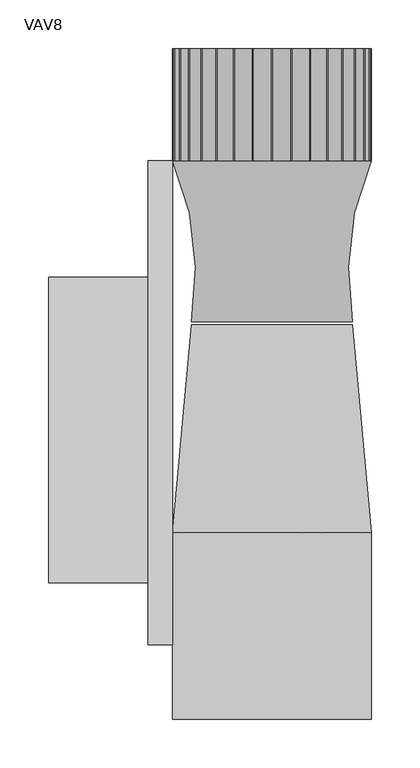
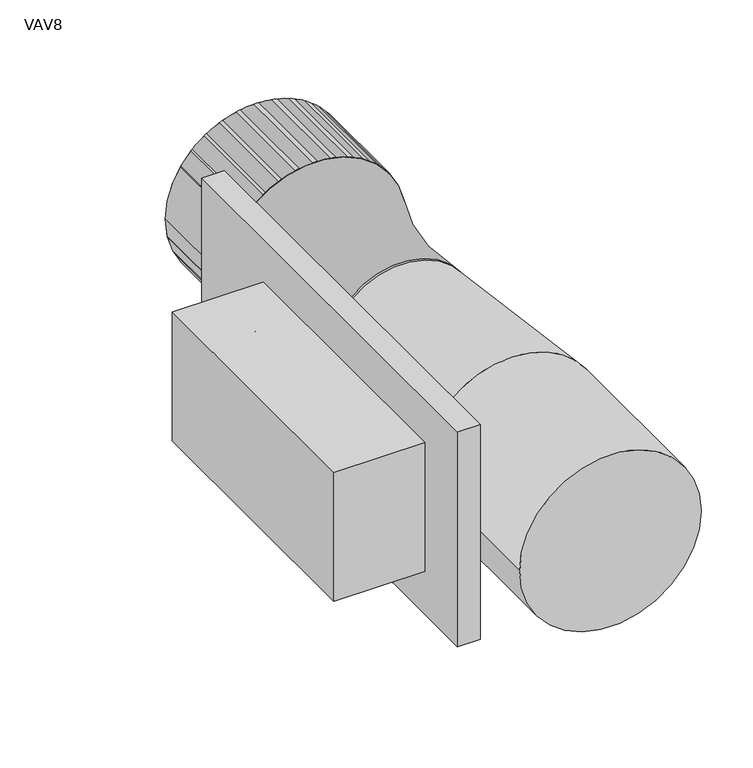
"""IFC4 building model written with IfcOpenShell, lengths in millimetres: proxy geometry, VAV8 : PValve200."""

import ifcopenshell
import ifcopenshell.guid

model = None  # the IFC model being written
_history = None  # IfcOwnerHistory: only IFC2X3 demands one
_inside = {}  # id of a spatial element -> (the spatial element, [elements in it])
_under = {}  # id of a project, library or spatial element -> (it, [spatial elements below it])
_declared = {}  # id of a project -> (the project, [libraries it declares])
_typed = {}  # id of a type object -> (the type object, [elements of that type])
_made_of = {}  # id of a material, layer set ... -> (it, [elements and type objects made of it])


def new_model(schema):
    """Start an empty IFC model of exactly this schema.

    Asked for "IFC4X3", IfcOpenShell would pick the latest addendum, in which some entities
    have other attributes; the version numbers below select the first issue.
    IFC2X3 requires an IfcOwnerHistory on every rooted entity: one is made here for all.
    """
    global model, _history
    if schema == "IFC4X3":
        model = ifcopenshell.file(schema_version=(4, 3, 0, 0))
    else:
        model = ifcopenshell.file(schema=schema)
    _inside.clear()
    _under.clear()
    _declared.clear()
    _typed.clear()
    _made_of.clear()
    _history = None
    if model.schema == "IFC2X3":
        org = make("IfcOrganization", Name="unknown")
        user = make(
            "IfcPersonAndOrganization",
            ThePerson=make("IfcPerson", FamilyName="unknown"),
            TheOrganization=org,
        )
        app = make(
            "IfcApplication",
            ApplicationDeveloper=org,
            Version="unknown",
            ApplicationFullName="unknown",
            ApplicationIdentifier="unknown",
        )
        _history = make(
            "IfcOwnerHistory",
            OwningUser=user,
            OwningApplication=app,
            ChangeAction="ADDED",
            CreationDate=0,
        )
    return model


def make(cls, **values):
    """One entity of the class cls with the attributes given. An attribute that is None is left unset."""
    return model.create_entity(
        cls, **{name: value for name, value in values.items() if value is not None}
    )


def rooted(cls, **values):
    """An entity with a GlobalId (a new one), such as an element, a storey or a relation."""
    return make(cls, GlobalId=ifcopenshell.guid.new(), OwnerHistory=_history, **values)


def si_unit(unit_type, name, prefix=None):
    """IfcSIUnit, for example si_unit("LENGTHUNIT", "METRE", prefix="MILLI")."""
    return make("IfcSIUnit", UnitType=unit_type, Prefix=prefix, Name=name)


def assignment(units):
    """IfcUnitAssignment: the units of a project."""
    return None if units is None else make("IfcUnitAssignment", Units=units)


def point(xyz):
    """IfcCartesianPoint."""
    return None if xyz is None else make("IfcCartesianPoint", Coordinates=xyz)


def direction(xyz):
    """IfcDirection."""
    return None if xyz is None else make("IfcDirection", DirectionRatios=xyz)


def frame(location, z_axis=None, x_axis=None):
    """IfcAxis2Placement3D, a coordinate frame: its origin and axes. An axis left out is left unset."""
    return make(
        "IfcAxis2Placement3D",
        Location=point(location),
        Axis=direction(z_axis),
        RefDirection=direction(x_axis),
    )


def frame_2d(location, x_axis=None):
    """IfcAxis2Placement2D, a coordinate frame in the plane: its origin and x axis."""
    return make(
        "IfcAxis2Placement2D", Location=point(location), RefDirection=direction(x_axis)
    )


def origin():
    """The frame at (0, 0, 0) with its axes left unset."""
    return frame((0.0, 0.0, 0.0))


def origin_2d():
    """The frame at (0, 0) in the plane with its x axis left unset."""
    return frame_2d((0.0, 0.0))


def place(relative_to, where):
    """IfcLocalPlacement: puts the frame where relative to a parent placement (None: the world)."""
    return make(
        "IfcLocalPlacement", PlacementRelTo=relative_to, RelativePlacement=where
    )


def context(
    kind, dimensions, precision=None, world=None, true_north=None, identifier=None
):
    """IfcGeometricRepresentationContext, for example the 3D "Model" context."""
    return make(
        "IfcGeometricRepresentationContext",
        ContextIdentifier=identifier,
        ContextType=kind,
        CoordinateSpaceDimension=dimensions,
        Precision=precision,
        WorldCoordinateSystem=world,
        TrueNorth=true_north,
    )


def project(units=None, contexts=None):
    """IfcProject with its units and contexts."""
    return rooted(
        "IfcProject",
        Name="project",
        RepresentationContexts=contexts,
        UnitsInContext=assignment(units),
    )


def spatial(cls, under=None, at=None, **own):
    """A site, building, storey or space (cls), placed at a placement, below another one or the project."""
    s = rooted(cls, ObjectPlacement=at, **own)
    if under is not None:
        _under.setdefault(under.id(), (under, []))[1].append(s)
    return s


def polyline(points):
    """IfcPolyline through the points."""
    return make("IfcPolyline", Points=[point(p) for p in points])


def circle_curve(where, radius):
    """IfcCircle in the frame where."""
    return make("IfcCircle", Position=where, Radius=radius)


def ellipse_curve(where, semi_axis1, semi_axis2):
    """IfcEllipse in the frame where."""
    return make(
        "IfcEllipse", Position=where, SemiAxis1=semi_axis1, SemiAxis2=semi_axis2
    )


def trimmed(basis, trim1, trim2, sense, master):
    """IfcTrimmedCurve: the piece of a basis curve between two trims."""
    return make(
        "IfcTrimmedCurve",
        BasisCurve=basis,
        Trim1=trim1,
        Trim2=trim2,
        SenseAgreement=sense,
        MasterRepresentation=master,
    )


def segment(curve, same_sense, transition):
    """IfcCompositeCurveSegment."""
    return make(
        "IfcCompositeCurveSegment",
        Transition=transition,
        SameSense=same_sense,
        ParentCurve=curve,
    )


def composite_curve(segments, self_intersect=None):
    """IfcCompositeCurve: segments joined end to end."""
    return make("IfcCompositeCurve", Segments=segments, SelfIntersect=self_intersect)


def outline(outer, holes=None, kind="AREA"):
    """IfcArbitraryClosedProfileDef: a profile drawn as a closed curve; with holes, ...WithVoids."""
    if holes is None:
        return make("IfcArbitraryClosedProfileDef", ProfileType=kind, OuterCurve=outer)
    return make(
        "IfcArbitraryProfileDefWithVoids",
        ProfileType=kind,
        OuterCurve=outer,
        InnerCurves=holes,
    )


def extrude(swept, where, along, depth):
    """IfcExtrudedAreaSolid: the profile swept, set in the frame where, extruded along a direction by depth."""
    return make(
        "IfcExtrudedAreaSolid",
        SweptArea=swept,
        Position=where,
        ExtrudedDirection=direction(along),
        Depth=depth,
    )


def shape(context_of_items, identifier, shape_type, items):
    """IfcShapeRepresentation: the items that make up one representation, for example the "Body"."""
    return make(
        "IfcShapeRepresentation",
        ContextOfItems=context_of_items,
        RepresentationIdentifier=identifier,
        RepresentationType=shape_type,
        Items=items,
    )


def source(mapping_origin, context_of_items, identifier, shape_type, items):
    """IfcRepresentationMap: a shape defined once, which mapped items show again and again."""
    return make(
        "IfcRepresentationMap",
        MappingOrigin=mapping_origin,
        MappedRepresentation=shape(context_of_items, identifier, shape_type, items),
    )


def transform(
    local_origin,
    x_axis=None,
    y_axis=None,
    z_axis=None,
    scale=None,
    scale2=None,
    scale3=None,
    uniform=True,
):
    """IfcCartesianTransformationOperator3D, or its non-uniform kind. x_axis, y_axis, z_axis: its Axis1, 2, 3."""
    if uniform:
        return make(
            "IfcCartesianTransformationOperator3D",
            Axis1=direction(x_axis),
            Axis2=direction(y_axis),
            LocalOrigin=point(local_origin),
            Scale=scale,
            Axis3=direction(z_axis),
        )
    return make(
        "IfcCartesianTransformationOperator3DnonUniform",
        Axis1=direction(x_axis),
        Axis2=direction(y_axis),
        LocalOrigin=point(local_origin),
        Scale=scale,
        Axis3=direction(z_axis),
        Scale2=scale2,
        Scale3=scale3,
    )


def mapped(mapping_source, mapping_target):
    """IfcMappedItem: shows the shape of a source again, moved by a transform."""
    return make(
        "IfcMappedItem", MappingSource=mapping_source, MappingTarget=mapping_target
    )


def made_of(thing, what):
    """Note that an element or type object is made of a material, layer set ...; save() writes the relation."""
    if what is not None:
        _made_of.setdefault(what.id(), (what, []))[1].append(thing)
    return thing


def element(
    cls,
    number,
    at=None,
    inside=None,
    cuts=None,
    type_object=None,
    material=None,
    context=None,
    identifier="Body",
    shape_type=None,
    held_by="IfcProductDefinitionShape",
    body=None,
    shapes=None,
    **own,
):
    """One element of the class cls, such as IfcWall. Its Tag is "e" and its number.

    at: its placement. inside: the storey or other place that contains it. cuts: it is an
    opening in that element (IfcRelVoidsElement). A single representation is given by context,
    identifier, shape_type and body (its items); several are given by shapes. held_by: the class
    of the entity that holds the representations. save() writes the other relations.
    """
    e = rooted(cls, Tag="e%d" % number, ObjectPlacement=at, **own)
    if body is not None:
        shapes = [shape(context, identifier, shape_type, body)]
    if shapes is not None:
        e.Representation = make(held_by, Representations=shapes)
    if inside is not None:
        _inside.setdefault(inside.id(), (inside, []))[1].append(e)
    if cuts is not None:
        rooted(
            "IfcRelVoidsElement", RelatingBuildingElement=cuts, RelatedOpeningElement=e
        )
    if type_object is not None:
        _typed.setdefault(type_object.id(), (type_object, []))[1].append(e)
    return made_of(e, material)


def aggregate(whole, parts):
    """IfcRelAggregates: a whole, such as a stair, and the parts it consists of."""
    return rooted("IfcRelAggregates", RelatingObject=whole, RelatedObjects=parts)


def save(model, path):
    """Write the relations noted so far, then the file.

    IfcRelAggregates (storeys below a building ...), IfcRelContainedInSpatialStructure (elements
    in a storey), IfcRelDefinesByType, IfcRelAssociatesMaterial and IfcRelDeclares: one each for
    every whole, place, type object, material and project.
    """
    for whole, parts in _under.values():
        aggregate(whole, parts)
    for where, things in _inside.values():
        rooted(
            "IfcRelContainedInSpatialStructure",
            RelatedElements=things,
            RelatingStructure=where,
        )
    for kind, things in _typed.values():
        rooted("IfcRelDefinesByType", RelatedObjects=things, RelatingType=kind)
    for what, things in _made_of.values():
        rooted("IfcRelAssociatesMaterial", RelatedObjects=things, RelatingMaterial=what)
    for by, libraries in _declared.values():
        rooted("IfcRelDeclares", RelatingContext=by, RelatedDefinitions=libraries)
    model.write(path)


def plane_surface(at):
    """IfcPlane: the flat surface through the origin of the frame at, square to its z axis."""
    return make("IfcPlane", Position=at)


def revolved_surface(curve, axis_point, axis_direction):
    """IfcSurfaceOfRevolution: the curve turned about the line through axis_point along axis_direction."""
    return make(
        "IfcSurfaceOfRevolution",
        SweptCurve=make("IfcArbitraryOpenProfileDef", ProfileType="CURVE", Curve=curve),
        AxisPosition=make("IfcAxis1Placement", Location=point(axis_point), Axis=direction(axis_direction)),
    )


def advanced_brep(points, edges, surfaces, faces):
    """IfcAdvancedBrep: a solid bounded by faces that lie on surfaces and meet in shared edges.

    An edge is (start, end): straight between two places in points (the first is 0);
    or (start, end, curve); or (start, end, curve, False) where it runs against its curve.
    A face is (place in surfaces, loops), or (place, loops, False) where it looks against
    its surface's normal. A loop lists edges by number (the first is 1), with a minus sign
    where the edge is run from its end to its start. The first loop is the outer one.
    """
    corners = [point(p) for p in points]
    vertices = [make("IfcVertexPoint", VertexGeometry=c) for c in corners]
    made = []
    for start, end, *more in edges:
        made.append(
            make(
                "IfcEdgeCurve",
                EdgeStart=vertices[start],
                EdgeEnd=vertices[end],
                EdgeGeometry=more[0] if more else make("IfcPolyline", Points=[corners[start], corners[end]]),
                SameSense=more[1] if len(more) > 1 else True,
            )
        )
    hull = []
    for where, loops, *sense in faces:
        bounds = []
        for j, loop in enumerate(loops):
            ring = [make("IfcOrientedEdge", EdgeElement=made[abs(k) - 1], Orientation=k > 0) for k in loop]
            bounds.append(
                make(
                    "IfcFaceOuterBound" if j == 0 else "IfcFaceBound",
                    Bound=make("IfcEdgeLoop", EdgeList=ring),
                    Orientation=True,
                )
            )
        hull.append(make("IfcAdvancedFace", Bounds=bounds, FaceSurface=surfaces[where], SameSense=sense[0] if sense else True))
    return make("IfcAdvancedBrep", Outer=make("IfcClosedShell", CfsFaces=hull))


def vav8_9bf4b91b(model_context):
    return source(origin(), model_context, "Body", "SolidModel", [
        extrude(outline(composite_curve([segment(trimmed(circle_curve(origin_2d(), 101.6), [point((0.0, 101.6))], [point((0.0, -101.6))], False, "CARTESIAN"), True, "CONTINUOUS"), segment(trimmed(circle_curve(origin_2d(), 101.6), [point((0.0, -101.6))], [point((0.0, 101.6))], False, "CARTESIAN"), True, "CONTINUOUS")], self_intersect=False)), frame((0.0, -114.3, 0.0), z_axis=(0.0, 1.0, 0.0), x_axis=(0.0, 0.0, 1.0)), (0.0, 0.0, 1.0), 114.3),
        advanced_brep(
        [(101.6, -114.3, 0.0), (-101.6, -114.3, 0.0), (-63.5, -114.3, 0.0), (63.5, -114.3, 0.0), (-82.55, -279.4, 0.0), (82.55, -279.4, 0.0), (63.5, -279.4, 0.0), (-63.5, -279.4, 0.0)],
        [
            (0, 1, circle_curve(frame((0.0, -114.3, 0.0), z_axis=(0.0, 1.0, 0.0), x_axis=(1.0, 0.0, 0.0)), 101.6)),
            (1, 2),
            (2, 3, circle_curve(frame((0.0, -114.3, 0.0), z_axis=(0.0, -1.0, 0.0), x_axis=(1.0, 0.0, 0.0)), 63.5)),
            (3, 0),
            (1, 0, circle_curve(frame((0.0, -114.3, 0.0), z_axis=(0.0, 1.0, 0.0), x_axis=(1.0, 0.0, 0.0)), 101.6)),
            (3, 2, circle_curve(frame((0.0, -114.3, 0.0), z_axis=(0.0, -1.0, 0.0), x_axis=(1.0, 0.0, 0.0)), 63.5)),
            (4, 5, circle_curve(frame((0.0, -279.4, 0.0), z_axis=(0.0, -1.0, 0.0), x_axis=(1.0, 0.0, 0.0)), 82.55)),
            (5, 6),
            (6, 7, circle_curve(frame((0.0, -279.4, 0.0), z_axis=(0.0, 1.0, 0.0), x_axis=(1.0, 0.0, 0.0)), 63.5)),
            (7, 4),
            (5, 4, circle_curve(frame((0.0, -279.4, 0.0), z_axis=(0.0, -1.0, 0.0), x_axis=(1.0, 0.0, 0.0)), 82.55)),
            (7, 6, circle_curve(frame((0.0, -279.4, 0.0), z_axis=(0.0, 1.0, 0.0), x_axis=(1.0, 0.0, 0.0)), 63.5)),
            (6, 3),
            (2, 7),
            (0, 5, circle_curve(frame((368.6011377, -228.756862, 0.0), z_axis=(0.0, 0.0, 1.0), x_axis=(1.0, 0.0, 0.0)), 290.4995367)),
            (4, 1, circle_curve(frame((-368.6011377, -228.756862, 0.0), z_axis=(0.0, 0.0, 1.0), x_axis=(-1.0, 0.0, 0.0)), 290.4995367)),
        ],
        [
            plane_surface(frame((0.0, -114.3, 0.0), z_axis=(0.0, 1.0, 0.0), x_axis=(1.0, 0.0, 0.0))),
            plane_surface(frame((0.0, -279.4, 0.0), z_axis=(0.0, -1.0, 0.0), x_axis=(1.0, 0.0, 0.0))),
            revolved_surface(polyline([(63.5, -279.4, 0.0), (63.5, -114.3, 0.0)]), (0.0, 0.0, 0.0), (0.0, -1.0, 0.0)),
            revolved_surface(trimmed(ellipse_curve(frame((368.6011377, -228.756862, 0.0), z_axis=(0.0, 0.0, -1.0), x_axis=(1.0, 0.0, 0.0)), 290.4995367, 290.4995367), [point((82.55, -279.4, 0.0))], [point((101.6, -114.3, 0.0))], True, "CARTESIAN"), (0.0, -114.3, 0.0), (0.0, 1.0, 0.0)),
        ],
        [
            (0, [[1, 2, 3, 4]]),
            (0, [[5, -4, 6, -2]]),
            (1, [[7, 8, 9, 10]]),
            (1, [[11, -10, 12, -8]]),
            (2, [[13, -3, 14, -9]]),
            (2, [[-13, -12, -14, -6]]),
            (3, [[-1, 15, -7, 16]]),
            (3, [[-5, -16, -11, -15]]),
        ],
    ),
        extrude(outline(composite_curve([segment(trimmed(circle_curve(origin_2d(), 101.6), [point((0.0, -101.6))], [point((0.0, 101.6))], False, "CARTESIAN"), True, "CONTINUOUS"), segment(trimmed(circle_curve(origin_2d(), 101.6), [point((0.0, 101.6))], [point((0.0, -101.6))], False, "CARTESIAN"), True, "CONTINUOUS")], self_intersect=False), holes=[composite_curve([segment(trimmed(circle_curve(origin_2d(), 63.5), [point((0.0, 63.5))], [point((0.0, -63.5))], True, "CARTESIAN"), True, "CONTINUOUS"), segment(trimmed(circle_curve(origin_2d(), 63.5), [point((0.0, -63.5))], [point((0.0, 63.5))], True, "CARTESIAN"), True, "CONTINUOUS")], self_intersect=False)]), frame((0.0, -114.3, 0.0), z_axis=(0.0, 1.0, 0.0), x_axis=(0.0, 0.0, 1.0)), (0.0, 0.0, 1.0), 114.3),
        extrude(outline(polyline([(-228.6, -546.1), (-228.6, -233.5601781), (-127.0, -233.5601781), (-127.0, -546.1), (-228.6, -546.1)])), frame((0.0, 0.0, -76.2), z_axis=(0.0, 0.0, 1.0), x_axis=(1.0, 0.0, 0.0)), (0.0, 0.0, 1.0), 152.4),
        extrude(outline(polyline([(-101.6, -609.6), (-127.0, -609.6), (-127.0, -114.3), (-101.6, -114.3), (-101.6, -609.6)])), frame((0.0, 0.0, -127.0), z_axis=(0.0, 0.0, 1.0), x_axis=(1.0, 0.0, 0.0)), (0.0, 0.0, 1.0), 254.0),
        extrude(outline(composite_curve([segment(trimmed(circle_curve(origin_2d(), 101.6), [point((0.0, -101.6))], [point((0.0, 101.6))], False, "CARTESIAN"), True, "CONTINUOUS"), segment(trimmed(circle_curve(origin_2d(), 101.6), [point((0.0, 101.6))], [point((0.0, -101.6))], False, "CARTESIAN"), True, "CONTINUOUS")], self_intersect=False)), frame((0.0, -685.8, 0.0), z_axis=(0.0, 1.0, 0.0), x_axis=(0.0, 0.0, 1.0)), (0.0, 0.0, 1.0), 190.5),
        advanced_brep(
        [(0.0, -495.3, 0.0), (-101.6, -495.3, 0.0), (101.6, -495.3, 0.0), (82.55, -282.3810845, 0.0), (-82.55, -282.3810845, 0.0), (0.0, -282.3810845, 0.0)],
        [
            (0, 1),
            (1, 2, circle_curve(frame((0.0, -495.3, 0.0), z_axis=(0.0, -1.0, 0.0), x_axis=(-1.0, 0.0, 0.0)), 101.6)),
            (2, 0),
            (2, 1, circle_curve(frame((0.0, -495.3, 0.0), z_axis=(0.0, -1.0, 0.0), x_axis=(-1.0, 0.0, 0.0)), 101.6)),
            (3, 4, circle_curve(frame((0.0, -282.3810845, 0.0), z_axis=(0.0, 1.0, 0.0), x_axis=(-1.0, 0.0, 0.0)), 82.55)),
            (4, 5),
            (5, 3),
            (4, 3, circle_curve(frame((0.0, -282.3810845, 0.0), z_axis=(0.0, 1.0, 0.0), x_axis=(-1.0, 0.0, 0.0)), 82.55)),
            (1, 4),
            (3, 2),
        ],
        [
            plane_surface(frame((0.0, -495.3, 0.0), z_axis=(0.0, -1.0, 0.0), x_axis=(-1.0, 0.0, 0.0))),
            plane_surface(frame((0.0, -282.3810845, 0.0), z_axis=(0.0, 1.0, 0.0), x_axis=(-1.0, 0.0, 0.0))),
            revolved_surface(polyline([(-82.55, -282.3810845, 0.0), (-101.6, -495.3, 0.0)]), (0.0, -279.4, 0.0), (0.0, -1.0, 0.0)),
        ],
        [
            (0, [[1, 2, 3]]),
            (0, [[-3, 4, -1]]),
            (1, [[5, 6, 7]]),
            (1, [[8, -7, -6]]),
            (2, [[-2, 9, -5, 10]]),
            (2, [[-4, -10, -8, -9]]),
        ],
    ),
    ])


if __name__ == "__main__":
    model = new_model("IFC4")
    model_context = context("Model", 3, world=origin())
    ifc_project = project(units=[si_unit("LENGTHUNIT", "METRE", prefix="MILLI")], contexts=[model_context])
    site = spatial("IfcSite", under=ifc_project)
    building = spatial("IfcBuilding", under=site)
    placement = place(None, origin())
    vav8_shape = vav8_9bf4b91b(model_context)
    element("IfcBuildingElementProxy", 1, Name="VAV8 : PValve200", ObjectType="VAV8 : PValve200", at=placement, inside=building, context=model_context, shape_type="MappedRepresentation", body=[
        mapped(vav8_shape, transform((0.0, 0.0, 0.0), x_axis=(1.0, 0.0, 0.0), y_axis=(0.0, 1.0, 0.0), z_axis=(0.0, 0.0, 1.0))),
    ])
    save(model, "model.ifc")

# Revit data of these elements
# Type "VAV8 : PValve200"
#   DuctSAUP = 0"
#   DuctSADN = 0"
#   Assembly Code = ""
